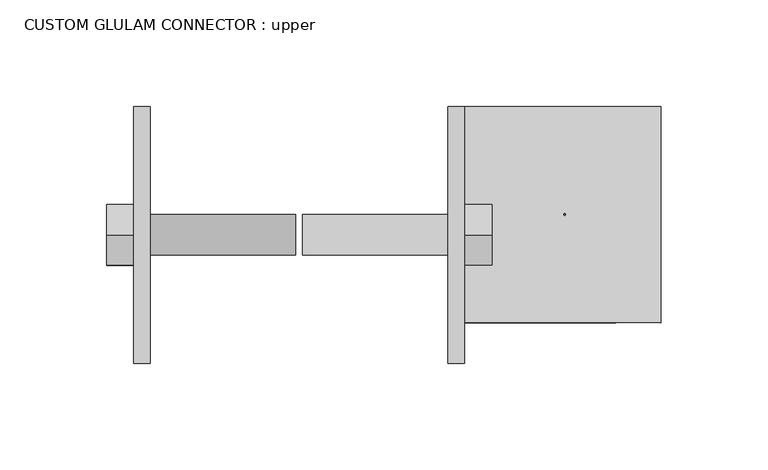
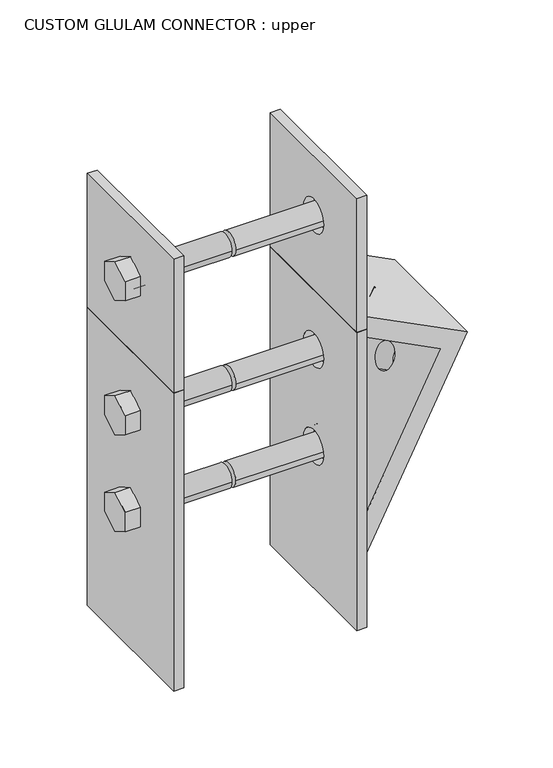
"""IFC4 building model written with IfcOpenShell, lengths in millimetres: fastener geometry, CUSTOM GLULAM CONNECTOR : upper."""

from ifc_helpers import new_model, si_unit, point, frame, frame_2d, origin, place, context, project, spatial, polyline, circle_curve, trimmed, segment, composite_curve, outline, extrude, source, transform, mapped, element, save
from ifc_brep_helpers import plane_surface, revolved_surface, advanced_brep


def custom_glulam_connector_upper_1e9803af(model_context):
    return source(origin(), model_context, "Body", "SolidModel", [
        advanced_brep(
        [(-77.7875, -60.325, 261.9375), (-69.85, -60.325, 261.9375), (-69.85, 60.325, 261.9375), (-77.7875, 60.325, 261.9375), (-77.7875, 52.3875, 261.9375), (-69.85, -60.325, 7.9375), (-69.85, 60.325, 7.9375), (-69.85, -13.890625, 211.1375), (-69.85, 13.890625, 211.1375), (-69.85, -13.890625, 128.5875), (-69.85, 13.890625, 128.5875), (-77.7875, -13.890625, 128.5875), (-77.7875, 13.890625, 128.5875), (-77.7875, 60.325, 7.9375), (-77.7875, 52.3875, 7.9375), (-77.7875, -60.325, 7.9375), (-77.7875, 13.890625, 211.1375), (-77.7875, -13.890625, 211.1375)],
        [
            (0, 1),
            (1, 2),
            (2, 3),
            (3, 4),
            (4, 0),
            (1, 5),
            (5, 6),
            (6, 2),
            (7, 8, circle_curve(frame((-69.85, 0.0, 211.1375), z_axis=(-1.0, 0.0, 0.0), x_axis=(0.0, 1.0, 0.0)), 13.890625)),
            (8, 7, circle_curve(frame((-69.85, 0.0, 211.1375), z_axis=(-1.0, 0.0, 0.0), x_axis=(0.0, 1.0, 0.0)), 13.890625)),
            (9, 10, circle_curve(frame((-69.85, 0.0, 128.5875), z_axis=(-1.0, 0.0, 0.0), x_axis=(0.0, 1.0, 0.0)), 13.890625)),
            (10, 9, circle_curve(frame((-69.85, 0.0, 128.5875), z_axis=(-1.0, 0.0, 0.0), x_axis=(0.0, 1.0, 0.0)), 13.890625)),
            (11, 12, circle_curve(frame((-77.7875, 0.0, 128.5875), z_axis=(-1.0, 0.0, 0.0), x_axis=(0.0, 1.0, 0.0)), 13.890625)),
            (12, 10),
            (9, 11),
            (3, 13),
            (13, 14),
            (14, 15),
            (15, 0),
            (16, 17, circle_curve(frame((-77.7875, 0.0, 211.1375), z_axis=(1.0, 0.0, 0.0), x_axis=(0.0, 1.0, 0.0)), 13.890625)),
            (17, 16, circle_curve(frame((-77.7875, 0.0, 211.1375), z_axis=(1.0, 0.0, 0.0), x_axis=(0.0, 1.0, 0.0)), 13.890625)),
            (11, 12, circle_curve(frame((-77.7875, 0.0, 128.5875), z_axis=(1.0, 0.0, 0.0), x_axis=(0.0, 1.0, 0.0)), 13.890625)),
            (15, 5),
            (6, 13),
            (8, 16),
            (17, 7),
        ],
        [
            plane_surface(frame((-77.7875, 60.325, 261.9375), z_axis=(0.0, 0.0, 1.0), x_axis=(1.0, 0.0, 0.0))),
            plane_surface(frame((-69.85, -60.325, 261.9375), z_axis=(1.0, 0.0, 0.0), x_axis=(0.0, 1.0, 0.0))),
            revolved_surface(polyline([(-77.7875, 13.890625, 128.5875), (-69.85, 13.890625, 128.5875)]), (-69.85, 0.0, 128.5875), (-1.0, 0.0, 0.0)),
            plane_surface(frame((-77.7875, -60.325, 261.9375), z_axis=(-1.0, 0.0, 0.0), x_axis=(0.0, -1.0, 0.0))),
            plane_surface(frame((-77.7875, -60.325, 261.9375), z_axis=(0.0, -1.0, 0.0), x_axis=(1.0, 0.0, 0.0))),
            plane_surface(frame((-77.7875, 60.325, 7.9375), z_axis=(0.0, 1.0, 0.0), x_axis=(1.0, 0.0, 0.0))),
            revolved_surface(polyline([(-77.7875, 13.890625, 211.1375), (-69.85, 13.890625, 211.1375)]), (-69.85, 0.0, 211.1375), (-1.0, 0.0, 0.0)),
            plane_surface(frame((-77.7875, -60.325, 7.9375), z_axis=(0.0, 0.0, -1.0), x_axis=(1.0, 0.0, 0.0))),
        ],
        [
            (0, [[1, 2, 3, 4, 5]]),
            (1, [[-2, 6, 7, 8], [9, 10], [11, 12]]),
            (2, [[13, 14, -11, 15]]),
            (3, [[16, 17, 18, 19, -5, -4], [20, 21], [-13, 22]]),
            (4, [[23, -6, -1, -19]]),
            (5, [[-3, -8, 24, -16]]),
            (6, [[-10, 25, -21, 26]]),
            (6, [[-20, -25, -9, -26]]),
            (2, [[-12, -14, -22, -15]]),
            (7, [[-24, -7, -23, -18, -17]]),
        ],
    ),
        extrude(outline(polyline([(-14.2875, 219.386392), (0.0, 227.6352839), (14.2875, 219.386392), (14.2875, 202.888608), (0.0, 194.6397161), (-14.2875, 202.888608), (-14.2875, 219.386392)])), frame((-90.4875, 0.0, 0.0), z_axis=(1.0, 0.0, 0.0), x_axis=(0.0, 1.0, 0.0)), (0.0, 0.0, 1.0), 12.7),
        extrude(outline(composite_curve([segment(trimmed(circle_curve(frame_2d((0.0, 211.1375)), 9.525), [point((-9.525, 211.1375))], [point((9.525, 211.1375))], False, "CARTESIAN"), True, "CONTINUOUS"), segment(trimmed(circle_curve(frame_2d((0.0, 211.1375)), 9.525), [point((9.525, 211.1375))], [point((-9.525, 211.1375))], False, "CARTESIAN"), True, "CONTINUOUS")], self_intersect=False)), frame((-77.7875, 0.0, 0.0), z_axis=(1.0, 0.0, 0.0), x_axis=(0.0, 1.0, 0.0)), (0.0, 0.0, 1.0), 76.2),
        extrude(outline(polyline([(-14.2875, 136.836392), (0.0, 145.0852839), (14.2875, 136.836392), (14.2875, 120.338608), (0.0, 112.0897161), (-14.2875, 120.338608), (-14.2875, 136.836392)])), frame((-90.4875, 0.0, 0.0), z_axis=(1.0, 0.0, 0.0), x_axis=(0.0, 1.0, 0.0)), (0.0, 0.0, 1.0), 12.7),
        extrude(outline(composite_curve([segment(trimmed(circle_curve(frame_2d((0.0, 128.5875)), 9.525), [point((-9.525, 128.5875))], [point((9.525, 128.5875))], False, "CARTESIAN"), True, "CONTINUOUS"), segment(trimmed(circle_curve(frame_2d((0.0, 128.5875)), 9.525), [point((9.525, 128.5875))], [point((-9.525, 128.5875))], False, "CARTESIAN"), True, "CONTINUOUS")], self_intersect=False)), frame((-77.7875, 0.0, 0.0), z_axis=(1.0, 0.0, 0.0), x_axis=(0.0, 1.0, 0.0)), (0.0, 0.0, 1.0), 76.2),
        extrude(outline(polyline([(-14.2875, 219.386392), (0.0, 227.6352839), (14.2875, 219.386392), (14.2875, 202.888608), (0.0, 194.6397161), (-14.2875, 202.888608), (-14.2875, 219.386392)])), frame((-90.4875, 0.0, 0.0), z_axis=(1.0, 0.0, 0.0), x_axis=(0.0, 1.0, 0.0)), (0.0, 0.0, 1.0), 12.7),
        extrude(outline(composite_curve([segment(trimmed(circle_curve(frame_2d((0.0, 211.1375)), 9.525), [point((-9.525, 211.1375))], [point((9.525, 211.1375))], False, "CARTESIAN"), True, "CONTINUOUS"), segment(trimmed(circle_curve(frame_2d((0.0, 211.1375)), 9.525), [point((9.525, 211.1375))], [point((-9.525, 211.1375))], False, "CARTESIAN"), True, "CONTINUOUS")], self_intersect=False)), frame((-77.7875, 0.0, 0.0), z_axis=(1.0, 0.0, 0.0), x_axis=(0.0, 1.0, 0.0)), (0.0, 0.0, 1.0), 76.2),
        advanced_brep(
        [(77.7875, -60.325, 261.9375), (77.7875, 52.3875, 261.9375), (77.7875, 60.325, 261.9375), (69.85, 60.325, 261.9375), (69.85, -60.325, 261.9375), (69.85, 60.325, 7.9375), (69.85, -60.325, 7.9375), (69.85, -13.890625, 211.1375), (69.85, 13.890625, 211.1375), (69.85, -13.890625, 128.5875), (69.85, 13.890625, 128.5875), (77.7875, -13.890625, 128.5875), (77.7875, 13.890625, 128.5875), (77.7875, -60.325, 7.9375), (77.7875, 52.3875, 7.9375), (77.7875, 60.325, 7.9375), (77.7875, 13.890625, 211.1375), (77.7875, -13.890625, 211.1375)],
        [
            (0, 1),
            (1, 2),
            (2, 3),
            (3, 4),
            (4, 0),
            (3, 5),
            (5, 6),
            (6, 4),
            (7, 8, circle_curve(frame((69.85, 0.0, 211.1375), z_axis=(1.0, 0.0, 0.0), x_axis=(0.0, 1.0, 0.0)), 13.890625)),
            (8, 7, circle_curve(frame((69.85, 0.0, 211.1375), z_axis=(1.0, 0.0, 0.0), x_axis=(0.0, 1.0, 0.0)), 13.890625)),
            (9, 10, circle_curve(frame((69.85, 0.0, 128.5875), z_axis=(1.0, 0.0, 0.0), x_axis=(0.0, 1.0, 0.0)), 13.890625)),
            (10, 9, circle_curve(frame((69.85, 0.0, 128.5875), z_axis=(1.0, 0.0, 0.0), x_axis=(0.0, 1.0, 0.0)), 13.890625)),
            (11, 9),
            (10, 12),
            (12, 11, circle_curve(frame((77.7875, 0.0, 128.5875), z_axis=(1.0, 0.0, 0.0), x_axis=(0.0, 1.0, 0.0)), 13.890625)),
            (0, 13),
            (13, 14),
            (14, 15),
            (15, 2),
            (16, 17, circle_curve(frame((77.7875, 0.0, 211.1375), z_axis=(-1.0, 0.0, 0.0), x_axis=(0.0, 1.0, 0.0)), 13.890625)),
            (17, 16, circle_curve(frame((77.7875, 0.0, 211.1375), z_axis=(-1.0, 0.0, 0.0), x_axis=(0.0, 1.0, 0.0)), 13.890625)),
            (12, 11, circle_curve(frame((77.7875, 0.0, 128.5875), z_axis=(-1.0, 0.0, 0.0), x_axis=(0.0, 1.0, 0.0)), 13.890625)),
            (6, 13),
            (15, 5),
            (7, 17),
            (16, 8),
        ],
        [
            plane_surface(frame((77.7875, 60.325, 261.9375), z_axis=(0.0, 0.0, 1.0), x_axis=(-1.0, 0.0, 0.0))),
            plane_surface(frame((69.85, -60.325, 261.9375), z_axis=(-1.0, 0.0, 0.0), x_axis=(0.0, 1.0, 0.0))),
            revolved_surface(polyline([(77.7875, 13.890625, 128.5875), (69.85, 13.890625, 128.5875)]), (69.85, 0.0, 128.5875), (1.0, 0.0, 0.0)),
            plane_surface(frame((77.7875, -60.325, 261.9375), z_axis=(1.0, 0.0, 0.0), x_axis=(0.0, -1.0, 0.0))),
            plane_surface(frame((77.7875, -60.325, 261.9375), z_axis=(0.0, -1.0, 0.0), x_axis=(-1.0, 0.0, 0.0))),
            plane_surface(frame((77.7875, 60.325, 7.9375), z_axis=(0.0, 1.0, 0.0), x_axis=(-1.0, 0.0, 0.0))),
            revolved_surface(polyline([(77.7875, 13.890625, 211.1375), (69.85, 13.890625, 211.1375)]), (69.85, 0.0, 211.1375), (1.0, 0.0, 0.0)),
            plane_surface(frame((77.7875, -60.325, 7.9375), z_axis=(0.0, 0.0, -1.0), x_axis=(-1.0, 0.0, 0.0))),
        ],
        [
            (0, [[1, 2, 3, 4, 5]]),
            (1, [[6, 7, 8, -4], [9, 10], [11, 12]]),
            (2, [[13, -12, 14, 15]]),
            (3, [[-2, -1, 16, 17, 18, 19], [20, 21], [22, -15]]),
            (4, [[-16, -5, -8, 23]]),
            (5, [[-19, 24, -6, -3]]),
            (6, [[25, -20, 26, -9]]),
            (6, [[-25, -10, -26, -21]]),
            (2, [[-13, -22, -14, -11]]),
            (7, [[-18, -17, -23, -7, -24]]),
        ],
    ),
        extrude(outline(polyline([(-14.2875, 219.386392), (0.0, 227.6352839), (14.2875, 219.386392), (14.2875, 202.888608), (0.0, 194.6397161), (-14.2875, 202.888608), (-14.2875, 219.386392)])), frame((77.7875, 0.0, 0.0), z_axis=(1.0, 0.0, 0.0), x_axis=(0.0, 1.0, 0.0)), (0.0, 0.0, 1.0), 12.7),
        extrude(outline(composite_curve([segment(trimmed(circle_curve(frame_2d((0.0, 211.1375)), 9.525), [point((-9.525, 211.1375))], [point((9.525, 211.1375))], False, "CARTESIAN"), True, "CONTINUOUS"), segment(trimmed(circle_curve(frame_2d((0.0, 211.1375)), 9.525), [point((9.525, 211.1375))], [point((-9.525, 211.1375))], False, "CARTESIAN"), True, "CONTINUOUS")], self_intersect=False)), frame((1.5875, 0.0, 0.0), z_axis=(1.0, 0.0, 0.0), x_axis=(0.0, 1.0, 0.0)), (0.0, 0.0, 1.0), 76.2),
        extrude(outline(polyline([(-14.2875, 136.836392), (0.0, 145.0852839), (14.2875, 136.836392), (14.2875, 120.338608), (0.0, 112.0897161), (-14.2875, 120.338608), (-14.2875, 136.836392)])), frame((77.7875, 0.0, 0.0), z_axis=(1.0, 0.0, 0.0), x_axis=(0.0, 1.0, 0.0)), (0.0, 0.0, 1.0), 12.7),
        extrude(outline(composite_curve([segment(trimmed(circle_curve(frame_2d((0.0, 128.5875)), 9.525), [point((-9.525, 128.5875))], [point((9.525, 128.5875))], False, "CARTESIAN"), True, "CONTINUOUS"), segment(trimmed(circle_curve(frame_2d((0.0, 128.5875)), 9.525), [point((9.525, 128.5875))], [point((-9.525, 128.5875))], False, "CARTESIAN"), True, "CONTINUOUS")], self_intersect=False)), frame((1.5875, 0.0, 0.0), z_axis=(1.0, 0.0, 0.0), x_axis=(0.0, 1.0, 0.0)), (0.0, 0.0, 1.0), 76.2),
        extrude(outline(polyline([(-14.2875, 219.386392), (0.0, 227.6352839), (14.2875, 219.386392), (14.2875, 202.888608), (0.0, 194.6397161), (-14.2875, 202.888608), (-14.2875, 219.386392)])), frame((77.7875, 0.0, 0.0), z_axis=(1.0, 0.0, 0.0), x_axis=(0.0, 1.0, 0.0)), (0.0, 0.0, 1.0), 12.7),
        extrude(outline(composite_curve([segment(trimmed(circle_curve(frame_2d((0.0, 211.1375)), 9.525), [point((-9.525, 211.1375))], [point((9.525, 211.1375))], False, "CARTESIAN"), True, "CONTINUOUS"), segment(trimmed(circle_curve(frame_2d((0.0, 211.1375)), 9.525), [point((9.525, 211.1375))], [point((-9.525, 211.1375))], False, "CARTESIAN"), True, "CONTINUOUS")], self_intersect=False)), frame((1.5875, 0.0, 0.0), z_axis=(1.0, 0.0, 0.0), x_axis=(0.0, 1.0, 0.0)), (0.0, 0.0, 1.0), 76.2),
        advanced_brep(
        [(-77.7875, -13.890625, 325.4375), (-77.7875, 13.890625, 325.4375), (-69.85, 13.890625, 325.4375), (-69.85, -13.890625, 325.4375), (-77.7875, 60.325, 376.2375), (-77.7875, 60.325, 261.9375), (-77.7875, -52.3875, 261.9375), (-77.7875, -60.325, 261.9375), (-77.7875, -60.325, 376.2375), (-69.85, -60.325, 261.9375), (-69.85, -60.325, 376.2375), (-69.85, 60.325, 376.2375), (-69.85, 60.325, 261.9375)],
        [
            (0, 1, circle_curve(frame((-77.7875, 0.0, 325.4375), z_axis=(-1.0, 0.0, 0.0), x_axis=(0.0, 1.0, 0.0)), 13.890625)),
            (1, 2),
            (2, 3, circle_curve(frame((-69.85, 0.0, 325.4375), z_axis=(1.0, 0.0, 0.0), x_axis=(0.0, 1.0, 0.0)), 13.890625)),
            (3, 0),
            (4, 5),
            (5, 6),
            (6, 7),
            (7, 8),
            (8, 4),
            (0, 1, circle_curve(frame((-77.7875, 0.0, 325.4375), z_axis=(1.0, 0.0, 0.0), x_axis=(0.0, 1.0, 0.0)), 13.890625)),
            (7, 9),
            (9, 10),
            (10, 8),
            (4, 11),
            (11, 12),
            (12, 5),
            (3, 2, circle_curve(frame((-69.85, 0.0, 325.4375), z_axis=(1.0, 0.0, 0.0), x_axis=(0.0, 1.0, 0.0)), 13.890625)),
            (10, 11),
            (9, 12),
        ],
        [
            revolved_surface(polyline([(-77.7875, 13.890625, 325.4375), (-69.85, 13.890625, 325.4375)]), (-69.85, 0.0, 325.4375), (-1.0, 0.0, 0.0)),
            plane_surface(frame((-77.7875, -60.325, 376.2375), z_axis=(-1.0, 0.0, 0.0), x_axis=(0.0, -1.0, 0.0))),
            plane_surface(frame((-77.7875, -60.325, 376.2375), z_axis=(0.0, -1.0, 0.0), x_axis=(1.0, 0.0, 0.0))),
            plane_surface(frame((-77.7875, 60.325, 261.9375), z_axis=(0.0, 1.0, 0.0), x_axis=(1.0, 0.0, 0.0))),
            plane_surface(frame((-77.7875, 60.325, 376.2375), z_axis=(0.0, 0.0, 1.0), x_axis=(1.0, 0.0, 0.0))),
            plane_surface(frame((-69.85, -60.325, 376.2375), z_axis=(1.0, 0.0, 0.0), x_axis=(0.0, 1.0, 0.0))),
            plane_surface(frame((-77.7875, -60.325, 261.9375), z_axis=(0.0, 0.0, -1.0), x_axis=(1.0, 0.0, 0.0))),
        ],
        [
            (0, [[1, 2, 3, 4]]),
            (1, [[5, 6, 7, 8, 9], [-1, 10]]),
            (2, [[11, 12, 13, -8]]),
            (3, [[14, 15, 16, -5]]),
            (0, [[17, -2, -10, -4]]),
            (4, [[-13, 18, -14, -9]]),
            (5, [[-18, -12, 19, -15], [-3, -17]]),
            (6, [[-16, -19, -11, -7, -6]]),
        ],
    ),
        extrude(outline(polyline([(-14.2875, 333.686392), (0.0, 341.9352839), (14.2875, 333.686392), (14.2875, 317.188608), (0.0, 308.9397161), (-14.2875, 317.188608), (-14.2875, 333.686392)])), frame((-90.4875, 0.0, 0.0), z_axis=(1.0, 0.0, 0.0), x_axis=(0.0, 1.0, 0.0)), (0.0, 0.0, 1.0), 12.7),
        extrude(outline(composite_curve([segment(trimmed(circle_curve(frame_2d((0.0, 325.4375)), 9.525), [point((-9.525, 325.4375))], [point((9.525, 325.4375))], False, "CARTESIAN"), True, "CONTINUOUS"), segment(trimmed(circle_curve(frame_2d((0.0, 325.4375)), 9.525), [point((9.525, 325.4375))], [point((-9.525, 325.4375))], False, "CARTESIAN"), True, "CONTINUOUS")], self_intersect=False)), frame((-77.7875, 0.0, 0.0), z_axis=(1.0, 0.0, 0.0), x_axis=(0.0, 1.0, 0.0)), (0.0, 0.0, 1.0), 76.2),
        advanced_brep(
        [(77.7875, -13.890625, 325.4375), (69.85, -13.890625, 325.4375), (69.85, 13.890625, 325.4375), (77.7875, 13.890625, 325.4375), (77.7875, 60.325, 376.2375), (77.7875, -60.325, 376.2375), (77.7875, -60.325, 261.9375), (77.7875, -52.3875, 261.9375), (77.7875, 60.325, 261.9375), (69.85, -60.325, 376.2375), (69.85, -60.325, 261.9375), (69.85, 60.325, 261.9375), (69.85, 60.325, 376.2375)],
        [
            (0, 1),
            (1, 2, circle_curve(frame((69.85, 0.0, 325.4375), z_axis=(-1.0, 0.0, 0.0), x_axis=(0.0, 1.0, 0.0)), 13.890625)),
            (2, 3),
            (3, 0, circle_curve(frame((77.7875, 0.0, 325.4375), z_axis=(1.0, 0.0, 0.0), x_axis=(0.0, 1.0, 0.0)), 13.890625)),
            (4, 5),
            (5, 6),
            (6, 7),
            (7, 8),
            (8, 4),
            (3, 0, circle_curve(frame((77.7875, 0.0, 325.4375), z_axis=(-1.0, 0.0, 0.0), x_axis=(0.0, 1.0, 0.0)), 13.890625)),
            (5, 9),
            (9, 10),
            (10, 6),
            (8, 11),
            (11, 12),
            (12, 4),
            (2, 1, circle_curve(frame((69.85, 0.0, 325.4375), z_axis=(-1.0, 0.0, 0.0), x_axis=(0.0, 1.0, 0.0)), 13.890625)),
            (12, 9),
            (11, 10),
        ],
        [
            revolved_surface(polyline([(77.7875, 13.890625, 325.4375), (69.85, 13.890625, 325.4375)]), (69.85, 0.0, 325.4375), (1.0, 0.0, 0.0)),
            plane_surface(frame((77.7875, -60.325, 376.2375), z_axis=(1.0, 0.0, 0.0), x_axis=(0.0, -1.0, 0.0))),
            plane_surface(frame((77.7875, -60.325, 376.2375), z_axis=(0.0, -1.0, 0.0), x_axis=(-1.0, 0.0, 0.0))),
            plane_surface(frame((77.7875, 60.325, 261.9375), z_axis=(0.0, 1.0, 0.0), x_axis=(-1.0, 0.0, 0.0))),
            plane_surface(frame((77.7875, 60.325, 376.2375), z_axis=(0.0, 0.0, 1.0), x_axis=(-1.0, 0.0, 0.0))),
            plane_surface(frame((69.85, -60.325, 376.2375), z_axis=(-1.0, 0.0, 0.0), x_axis=(0.0, 1.0, 0.0))),
            plane_surface(frame((77.7875, -60.325, 261.9375), z_axis=(0.0, 0.0, -1.0), x_axis=(-1.0, 0.0, 0.0))),
        ],
        [
            (0, [[1, 2, 3, 4]]),
            (1, [[5, 6, 7, 8, 9], [10, -4]]),
            (2, [[-6, 11, 12, 13]]),
            (3, [[-9, 14, 15, 16]]),
            (0, [[-1, -10, -3, 17]]),
            (4, [[-5, -16, 18, -11]]),
            (5, [[-15, 19, -12, -18], [-17, -2]]),
            (6, [[-8, -7, -13, -19, -14]]),
        ],
    ),
        extrude(outline(polyline([(-14.2875, 333.686392), (0.0, 341.9352839), (14.2875, 333.686392), (14.2875, 317.188608), (0.0, 308.9397161), (-14.2875, 317.188608), (-14.2875, 333.686392)])), frame((77.7875, 0.0, 0.0), z_axis=(1.0, 0.0, 0.0), x_axis=(0.0, 1.0, 0.0)), (0.0, 0.0, 1.0), 12.7),
        extrude(outline(composite_curve([segment(trimmed(circle_curve(frame_2d((0.0, 325.4375)), 9.525), [point((-9.525, 325.4375))], [point((9.525, 325.4375))], False, "CARTESIAN"), True, "CONTINUOUS"), segment(trimmed(circle_curve(frame_2d((0.0, 325.4375)), 9.525), [point((9.525, 325.4375))], [point((-9.525, 325.4375))], False, "CARTESIAN"), True, "CONTINUOUS")], self_intersect=False)), frame((1.5875, 0.0, 0.0), z_axis=(1.0, 0.0, 0.0), x_axis=(0.0, 1.0, 0.0)), (0.0, 0.0, 1.0), 76.2),
        advanced_brep(
        [(170.0383695, -41.275, 215.9775257), (77.7875, -41.275, 262.9816915), (77.7875, -41.275, 245.1647625), (148.6865418, -41.275, 209.0398963), (77.7875, -41.275, 69.8926921), (77.7875, -41.275, 34.925), (170.0383695, 60.325, 215.9775257), (77.7875, 60.325, 34.925), (77.7875, 60.325, 69.8926921), (148.6865418, 60.325, 209.0398963), (77.7875, 60.325, 245.1647625), (77.7875, 60.325, 262.9816915), (125.1288563, 9.525, 238.8600656), (124.4216199, 9.525, 239.2204206), (117.2145207, 9.525, 225.075692), (117.9217571, 9.525, 224.7153371), (137.6957155, 9.525, 187.4691853), (127.9661316, 9.525, 168.3738017), (142.1108602, 9.525, 161.1667025), (151.8404441, 9.525, 180.2620861)],
        [
            (0, 1),
            (1, 2),
            (2, 3),
            (3, 4),
            (4, 5),
            (5, 0),
            (6, 7),
            (7, 8),
            (8, 9),
            (9, 10),
            (10, 11),
            (11, 6),
            (0, 6),
            (11, 1),
            (12, 13, circle_curve(frame((124.7752381, 9.525, 239.0402431), z_axis=(-0.45399049973954897, 0.0, -0.8910065241883668), x_axis=(-0.8910065241883668, 0.0, 0.45399049973954897)), 0.396875)),
            (13, 12, circle_curve(frame((124.7752381, 9.525, 239.0402431), z_axis=(-0.45399049973954897, 0.0, -0.8910065241883668), x_axis=(-0.8910065241883668, 0.0, 0.45399049973954897)), 0.396875)),
            (10, 2),
            (9, 3),
            (14, 15, circle_curve(frame((117.5681389, 9.525, 224.8955145), z_axis=(0.45399049973954897, 0.0, 0.8910065241883668), x_axis=(-0.8910065241883668, 0.0, 0.45399049973954897)), 0.396875)),
            (15, 14, circle_curve(frame((117.5681389, 9.525, 224.8955145), z_axis=(0.45399049973954897, 0.0, 0.8910065241883668), x_axis=(-0.8910065241883668, 0.0, 0.45399049973954897)), 0.396875)),
            (8, 4),
            (16, 17, circle_curve(frame((132.8309236, 9.525, 177.9214935), z_axis=(0.8910065241883661, 0.0, -0.4539904997395502), x_axis=(0.4539904997395502, 0.0, 0.8910065241883661)), 10.715625)),
            (17, 16, circle_curve(frame((132.8309236, 9.525, 177.9214935), z_axis=(0.8910065241883661, 0.0, -0.4539904997395502), x_axis=(0.4539904997395502, 0.0, 0.8910065241883661)), 10.715625)),
            (7, 5),
            (18, 19, circle_curve(frame((146.9756522, 9.525, 170.7143943), z_axis=(-0.8910065241883661, 0.0, 0.4539904997395502), x_axis=(0.4539904997395502, 0.0, 0.8910065241883661)), 10.715625)),
            (19, 18, circle_curve(frame((146.9756522, 9.525, 170.7143943), z_axis=(-0.8910065241883661, 0.0, 0.4539904997395502), x_axis=(0.4539904997395502, 0.0, 0.8910065241883661)), 10.715625)),
            (12, 15),
            (14, 13),
            (18, 17),
            (16, 19),
        ],
        [
            plane_surface(frame((77.7875, -41.275, 262.9816915), z_axis=(0.0, -1.0, 0.0), x_axis=(-0.8910065241883668, 0.0, 0.45399049973954897))),
            plane_surface(frame((77.7875, 60.325, 262.9816915), z_axis=(0.0, 1.0, 0.0), x_axis=(0.8910065241883668, 0.0, -0.45399049973954897))),
            plane_surface(frame((170.0383695, -41.275, 215.9775257), z_axis=(0.45399049973954897, 0.0, 0.8910065241883668), x_axis=(0.0, 1.0, 0.0))),
            plane_surface(frame((77.7875, -41.275, 262.9816915), z_axis=(-1.0, 0.0, 0.0), x_axis=(0.0, 1.0, 0.0))),
            plane_surface(frame((77.7875, -41.275, 245.1647625), z_axis=(-0.4539904997395488, 0.0, -0.8910065241883668), x_axis=(0.0, 1.0, 0.0))),
            plane_surface(frame((148.6865418, -41.275, 209.0398963), z_axis=(-0.8910065241883659, 0.0, 0.45399049973955063), x_axis=(0.0, 1.0, 0.0))),
            plane_surface(frame((77.7875, -41.275, 69.8926921), z_axis=(-1.0, 0.0, 0.0), x_axis=(0.0, 1.0, 0.0))),
            plane_surface(frame((77.7875, -41.275, 34.925), z_axis=(0.8910065241883661, 0.0, -0.4539904997395502), x_axis=(0.0, 1.0, 0.0))),
            revolved_surface(polyline([(117.21452068738647, 9.525, 225.0756919787313), (124.42161989691586, 9.525, 239.22042060157148)]), (124.7752381, 9.525, 239.0402431), (-0.45399049973954897, 0.0, -0.8910065241883668)),
            revolved_surface(polyline([(137.69571550343758, 9.525, 187.4691853067466), (151.84044414877164, 9.525, 180.26208608575598)]), (146.9756522, 9.525, 170.7143943), (-0.8910065241883661, 0.0, 0.4539904997395502)),
        ],
        [
            (0, [[1, 2, 3, 4, 5, 6]]),
            (1, [[7, 8, 9, 10, 11, 12]]),
            (2, [[-1, 13, -12, 14], [15, 16]]),
            (3, [[-2, -14, -11, 17]]),
            (4, [[-3, -17, -10, 18], [19, 20]]),
            (5, [[-4, -18, -9, 21], [22, 23]]),
            (6, [[-5, -21, -8, 24]]),
            (7, [[-6, -24, -7, -13], [25, 26]]),
            (8, [[27, -19, 28, -15]]),
            (8, [[-27, -16, -28, -20]]),
            (9, [[29, -22, 30, -25]]),
            (9, [[-29, -26, -30, -23]]),
        ],
    ),
    ])


if __name__ == "__main__":
    model = new_model("IFC4")
    model_context = context("Model", 3, world=origin())
    ifc_project = project(units=[si_unit("LENGTHUNIT", "METRE", prefix="MILLI")], contexts=[model_context])
    site = spatial("IfcSite", under=ifc_project)
    building = spatial("IfcBuilding", under=site)
    placement = place(None, origin())
    custom_glulam_connector_upper_shape = custom_glulam_connector_upper_1e9803af(model_context)
    element("IfcFastener", 1, ObjectType="CUSTOM GLULAM CONNECTOR : upper", at=placement, inside=building, context=model_context, shape_type="MappedRepresentation", body=[
        mapped(custom_glulam_connector_upper_shape, transform((0.0, 0.0, 0.0), x_axis=(1.0, 0.0, 0.0), y_axis=(0.0, 1.0, 0.0), z_axis=(0.0, 0.0, 1.0))),
    ])
    save(model, "model.ifc")

# Revit data of these elements
# Type "CUSTOM GLULAM CONNECTOR : upper"
#   Width - Top = 0' - 5 1/2"
#   Top/Bottom Plate Thickness = 0' - 0 5/16"
#   Top/Bottom Plate - Width = 0' - 7 1/2"
#   Rod Radius = 0' - 0 3/8"
#   Rod Length [instance default] = 1' - 0"
#   Plate Thickness = 0' - 0 5/16"
#   Offset - Upper Plate 2 = 0' - 0"
#   Height of Plate = 0' - 10"
#   Width - Bottom = 0' - 5 1/2"
#   Plate Width = 0' - 4 3/4"
#   Bracket Width = 0' - 4"
#   Bracket Thickness = 0' - 0 5/8"
#   Bracket Offset in X = 0' - 3 1/16"
#   Bracket Offset in Y = 0' - 0"
#   Bracket Offset = 0' - 1 3/8"
#   Bracket Leg = 0' - 8"
#   Bracket Hole Radius - Up = 0' - 0 1/64"
#   Bracket Hole Radius - Down = 0' - 0 27/64"
#   Bracket Hole Offset = 0' - 2"
#   Beam Width = 0' - 7 3/8"
#   Angle 2 = 63.00°
#   Angle 1 = 153.00°
#   Top Plate Visible = no
#   Rod Visibility = no
#   Plate Visibility - Upper Right 2 = no
#   Plate Visibility - Upper Right 1 = yes
#   Plate Visibility - Upper Left 2 = no
#   Plate Visibility - Upper Left 1 = yes
#   Plate Visibility - Lower Right 2 = no
#   Plate Visibility - Lower Right 1 = yes
#   Plate Visibility - Lower Left 2 = no
#   Plate Visibility - Lower Left 1 = yes
#   Bracket Visibility = yes
#   Bottom Plate Visible = no
#   Upper Plates - 2 = element 1407874
#   Upper Plates - 1 = element 1407868
#   Lower Plates = element 1407872
#   Bracket Material = 5/8" STEEL ANGLE (HDG AFTER FABRICATION)
#   URL = ""
# Element 1 (IfcFastener, "CUSTOM GLULAM CONNECTOR : upper")
#   Materials on its faces: "3/4\" LAG BOLT (THRU BOLT IF PLATE ON OPP. SIDE OF STRUCT MEMBER)", "5/16\" STEEL PLATE (HDG AFTER FABRICATION)", "5/8\" STEEL ANGLE (HDG AFTER FABRICATION)"
# Materials
#   "5/8\" STEEL ANGLE (HDG AFTER FABRICATION)": class "Generic", colour RGB 195 195 195, transparency 0, Cost = 0
#   "3/4\" LAG BOLT (THRU BOLT IF PLATE ON OPP. SIDE OF STRUCT MEMBER)": class "Generic", colour RGB 120 120 120, transparency 0, Cost = 0
#   "5/16\" STEEL PLATE (HDG AFTER FABRICATION)": class "Generic", colour RGB 232 232 232, transparency 0, Cost = 0
